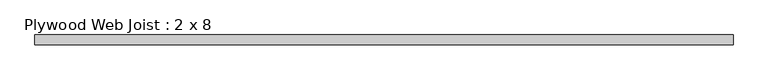
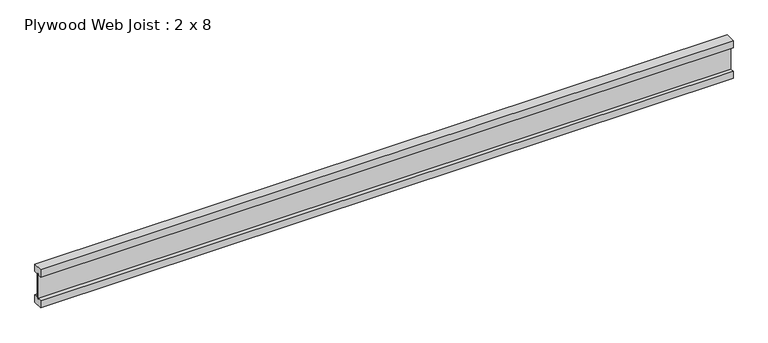
"""IFC4 building model written with IfcOpenShell, lengths in millimetres: beam geometry, Plywood Web Joist : 2 x 8."""

from ifc_helpers import new_model, si_unit, frame, origin, place, context, project, spatial, polyline, outline, extrude, source, transform, mapped, element, save


def plywood_web_joist_2_x_8_8e4157b3(model_context):
    return source(origin(), model_context, "Body", "SweptSolid", [
        extrude(outline(polyline([(-25.4, 101.6), (25.4, 101.6), (25.4, 63.5), (4.7625, 63.5), (4.7625, 69.85), (-4.7625, 69.85), (-4.7625, 63.5), (-25.4, 63.5), (-25.4, 101.6)])), frame((-1758.95, 0.0, 0.0), z_axis=(1.0, 0.0, 0.0), x_axis=(0.0, 1.0, 0.0)), (0.0, 0.0, 1.0), 3517.9),
        extrude(outline(polyline([(25.4, -63.5), (25.4, -101.6), (-25.4, -101.6), (-25.4, -63.5), (-4.7625, -63.5), (-4.7625, -69.1160374), (4.7625, -69.1160374), (4.7625, -63.5), (25.4, -63.5)])), frame((-1758.95, 0.0, 0.0), z_axis=(1.0, 0.0, 0.0), x_axis=(0.0, 1.0, 0.0)), (0.0, 0.0, 1.0), 3517.9),
        extrude(outline(polyline([(1758.95, 4.7625), (1758.95, -4.7625), (-1758.95, -4.7625), (-1758.95, 4.7625), (1758.95, 4.7625)])), frame((0.0, 0.0, -69.1160374), z_axis=(0.0, 0.0, 1.0), x_axis=(1.0, 0.0, 0.0)), (0.0, 0.0, 1.0), 138.9660374),
    ])


if __name__ == "__main__":
    model = new_model("IFC4")
    model_context = context("Model", 3, world=origin())
    ifc_project = project(units=[si_unit("LENGTHUNIT", "METRE", prefix="MILLI")], contexts=[model_context])
    site = spatial("IfcSite", under=ifc_project)
    building = spatial("IfcBuilding", under=site)
    placement = place(None, origin())
    plywood_web_joist_2_x_8_shape = plywood_web_joist_2_x_8_8e4157b3(model_context)
    element("IfcBeam", 1, ObjectType="Plywood Web Joist : 2 x 8", at=placement, inside=building, context=model_context, shape_type="MappedRepresentation", body=[
        mapped(plywood_web_joist_2_x_8_shape, transform((0.0, 0.0, 0.0), x_axis=(1.0, 0.0, 0.0), y_axis=(0.0, 1.0, 0.0), z_axis=(0.0, 0.0, 1.0))),
    ])
    save(model, "model.ifc")

# Revit data of these elements
# Type "Plywood Web Joist : 2 x 8"
#   Assembly Code = "B10"
#   Length [instance default] = 5' - 0"
#   b = 0' - 2"
#   d = 0' - 8"
#   Structural Material [instance default] = Softwood, Lumber
# Element 1 (IfcBeam, "Plywood Web Joist : 2 x 8")
#   Materials on its faces: "Softwood, Lumber"
# Materials
#   "Softwood, Lumber": class "Wood", colour RGB 144 113 62, transparency 0, Description = "Pinus Echinata", Cost = 0
